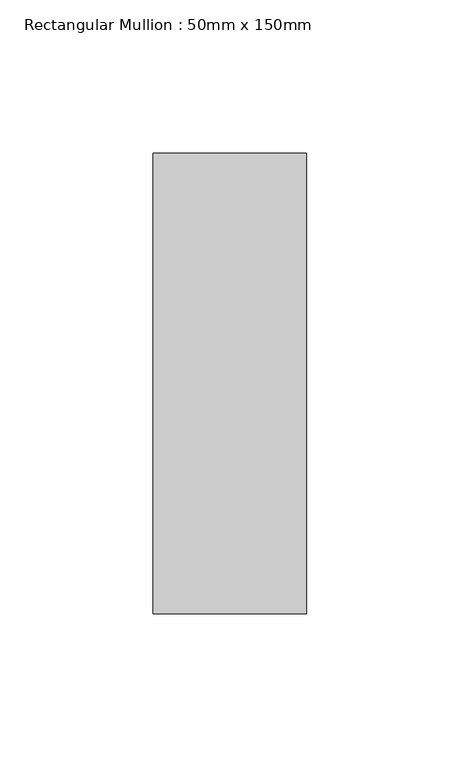
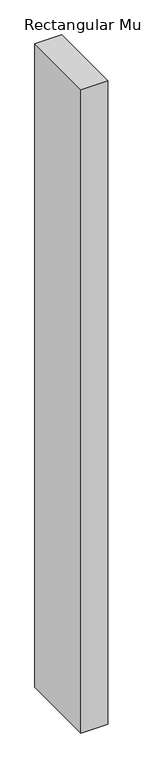
"""IFC4 building model written with IfcOpenShell, lengths in millimetres: member geometry, Rectangular Mullion : 50mm x 150mm."""

from ifc_helpers import new_model, si_unit, frame, origin, place, context, project, spatial, polyline, outline, extrude, source, transform, mapped, element, save


def rectangular_mullion_50mm_x_150mm_11a5ee59(model_context):
    return source(origin(), model_context, "Body", "SweptSolid", [
        extrude(outline(polyline([(0.0, 75.0), (0.0, -75.0), (-50.0, -75.0), (-50.0, 75.0), (0.0, 75.0)])), frame((0.0, 0.0, -1278.5714285), z_axis=(0.0, 0.0, 1.0), x_axis=(1.0, 0.0, 0.0)), (0.0, 0.0, 1.0), 1278.5714285),
    ])


if __name__ == "__main__":
    model = new_model("IFC4")
    model_context = context("Model", 3, world=origin())
    ifc_project = project(units=[si_unit("LENGTHUNIT", "METRE", prefix="MILLI")], contexts=[model_context])
    site = spatial("IfcSite", under=ifc_project)
    building = spatial("IfcBuilding", under=site)
    placement = place(None, origin())
    rectangular_mullion_50mm_x_150mm_shape = rectangular_mullion_50mm_x_150mm_11a5ee59(model_context)
    element("IfcMember", 1, ObjectType="Rectangular Mullion : 50mm x 150mm", at=placement, inside=building, context=model_context, shape_type="MappedRepresentation", body=[
        mapped(rectangular_mullion_50mm_x_150mm_shape, transform((0.0, 0.0, 0.0), x_axis=(1.0, 0.0, 0.0), y_axis=(0.0, 1.0, 0.0), z_axis=(0.0, 0.0, 1.0))),
    ])
    save(model, "model.ifc")

# Revit data of these elements
# Type "Rectangular Mullion : 50mm x 150mm"
#   built-in parameter 1007304 = 0.492126 (stored number, unit not read)
#   built-in parameter 1007301 = 0.082021 (stored number, unit not read)
#   built-in parameter 1007300 = 0.082021 (stored number, unit not read)
# Element 1 (IfcMember, "Rectangular Mullion : 50mm x 150mm")
#   Materials on its faces: "Aluminum"
# Materials
#   "Aluminum": class "Metal", colour RGB 247 247 247, transparency 0, Description = "Aluminum 6061", Cost = 0
